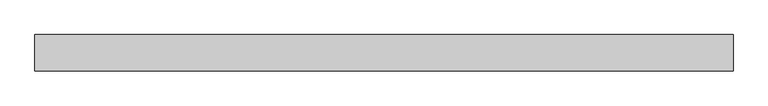
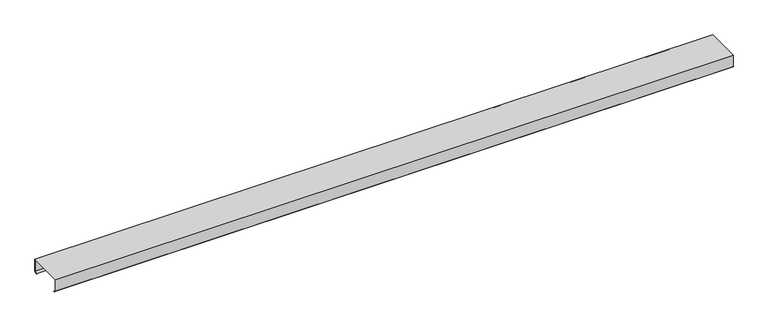
"""IFC4 building model written with IfcOpenShell, lengths in millimetres: proxy geometry, Generic Models 7:Generic Models 1:1:Generic Models 1:1 : Generic Models 7:Generic Models 1:337419:10 : Generic Models 7:Generic Models 1:1:Generic Models 1:1 : Generic Models 7:Generic Models 1:337419:306201."""

from ifc_helpers import new_model, si_unit, frame, origin, place, context, project, spatial, polyline, outline, extrude, source, transform, mapped, element, save


def generic_models_678c35c7(model_context):
    return source(origin(), model_context, "Body", "SweptSolid", [
        extrude(outline(polyline([(-568186.6413841, 2544.5640625), (-567932.6413841, 2544.5640625), (-567932.6413841, 2455.6640625), (-567947.2345307, 2443.4189586), (-567949.0202751, 2445.5471258), (-567935.4195091, 2456.9595235), (-567935.4195091, 2541.7859375), (-568183.8632591, 2541.7859375), (-568183.8632591, 2456.9595235), (-568170.2624931, 2445.5471258), (-568172.0482375, 2443.4189586), (-568186.6413841, 2455.6640625), (-568186.6413841, 2544.5640625)])), frame((591306.0367239, 0.0, 0.0), z_axis=(1.0, 0.0, 0.0), x_axis=(0.0, 1.0, 0.0)), (0.0, 0.0, 1.0), 4876.8),
    ])


if __name__ == "__main__":
    model = new_model("IFC4")
    model_context = context("Model", 3, world=origin())
    ifc_project = project(units=[si_unit("LENGTHUNIT", "METRE", prefix="MILLI")], contexts=[model_context])
    site = spatial("IfcSite", under=ifc_project)
    building = spatial("IfcBuilding", under=site)
    placement = place(None, origin())
    generic_models_shape = generic_models_678c35c7(model_context)
    element("IfcBuildingElementProxy", 1, Name="Generic Models 7:Generic Models 1:1:Generic Models 1:1 : Generic Models 7:Generic Models 1:337419:10 : Generic Models 7:Generic Models 1:1:Generic Models 1:1 : Generic Models 7:Generic Models 1:337419:306201", ObjectType="Generic Models 7:Generic Models 1:1:Generic Models 1:1 : Generic Models 7:Generic Models 1:337419:10 : Generic Models 7:Generic Models 1:1:Generic Models 1:1 : Generic Models 7:Generic Models 1:337419:306201", at=placement, inside=building, context=model_context, shape_type="MappedRepresentation", body=[
        mapped(generic_models_shape, transform((0.0, 0.0, 0.0), x_axis=(1.0, 0.0, 0.0), y_axis=(0.0, 1.0, 0.0), z_axis=(0.0, 0.0, 1.0))),
    ])
    save(model, "model.ifc")

# Revit data of these elements
# Type "Generic Models 7:Generic Models 1:1:Generic Models 1:1 : Generic Models 7:Generic Models 1:337419:10 : Generic Models 7:Generic Models 1:1:Generic Models 1:1 : Generic Models 7:Generic Models 1:337419:306201"
#   NameOverride = "Generic Models 7:Generic Models 1:1:Generic Models 1:1 : Generic Models 7:Generic Models 1:337419:306201"
#   ObjectTypeOverride = "Generic Models 1:1 : Generic Models 7:Generic Models 1:337419"
#   Reference = "Generic Models 1"
#   Tag = "306201"
# Element 1 (IfcBuildingElementProxy, "Generic Models 7:Generic Models 1:1:Generic Models 1:1 : Generic Models 7:Generic Models 1:337419:10 : Generic Models 7:Generic Models 1:1:Generic Models 1:1 : Generic Models 7:Generic Models 1:337419:306201")
#   Materials on its faces: "'ZEE' SECTION (8.0x3.5Z - SEE STRUCT. DWGS)"
# Materials
#   "'ZEE' SECTION (8.0x3.5Z - SEE STRUCT. DWGS)": class "Unassigned", colour RGB 210 209 208, transparency 0, Keynote = "M05121300.02", Cost = 0
